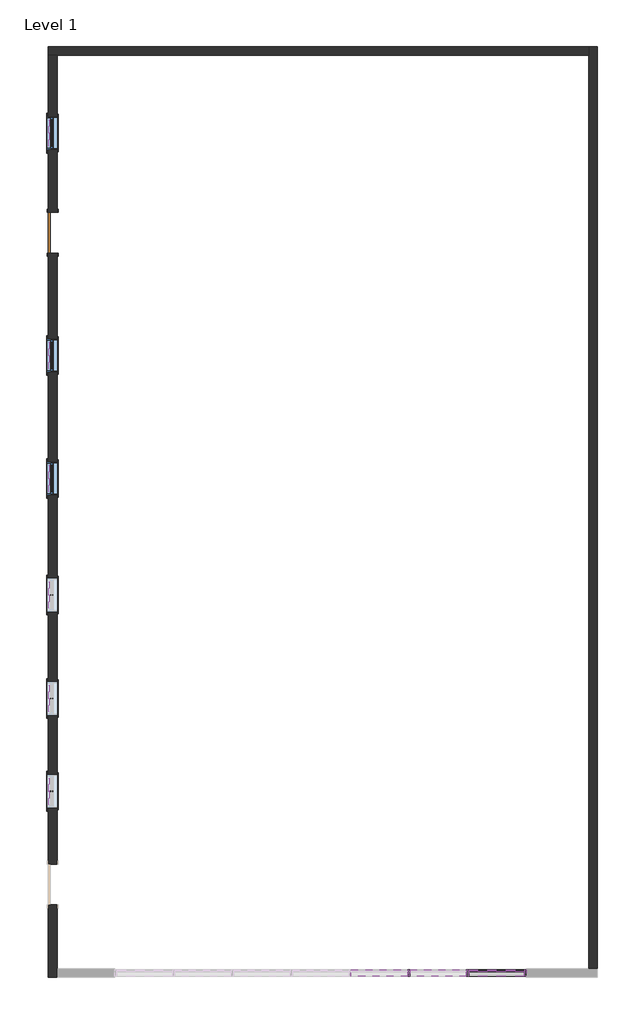
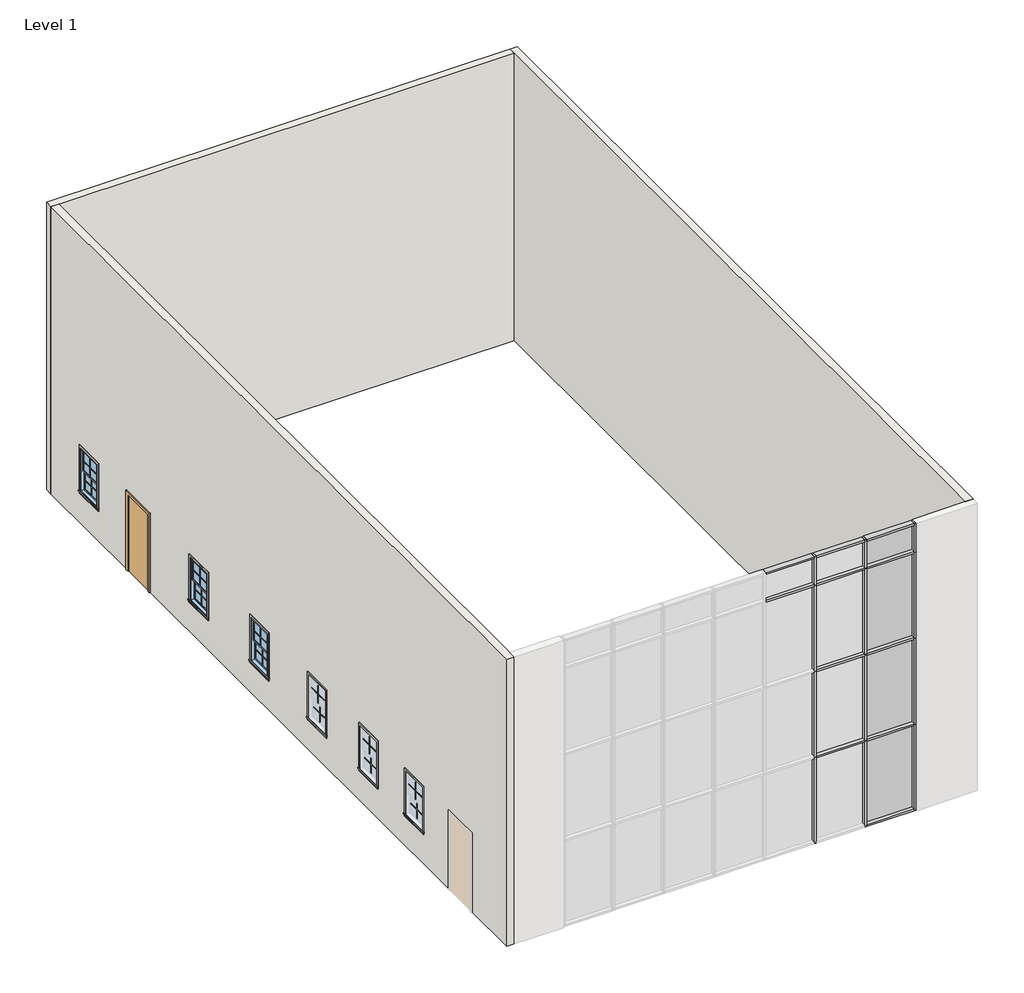
# One storey, part 2 of 2: 24 proxies, 23 members, 4 plates, 3 walls, 3 windows, 1 door.
"""IFC4 building model written with IfcOpenShell, lengths in millimetres."""

import ifcopenshell
import ifcopenshell.guid

model = None  # the IFC model being written
_history = None  # IfcOwnerHistory: only IFC2X3 demands one
_inside = {}  # id of a spatial element -> (the spatial element, [elements in it])
_under = {}  # id of a project, library or spatial element -> (it, [spatial elements below it])
_declared = {}  # id of a project -> (the project, [libraries it declares])
_typed = {}  # id of a type object -> (the type object, [elements of that type])
_made_of = {}  # id of a material, layer set ... -> (it, [elements and type objects made of it])


def new_model(schema):
    """Start an empty IFC model of exactly this schema.

    Asked for "IFC4X3", IfcOpenShell would pick the latest addendum, in which some entities
    have other attributes; the version numbers below select the first issue.
    IFC2X3 requires an IfcOwnerHistory on every rooted entity: one is made here for all.
    """
    global model, _history
    if schema == "IFC4X3":
        model = ifcopenshell.file(schema_version=(4, 3, 0, 0))
    else:
        model = ifcopenshell.file(schema=schema)
    _inside.clear()
    _under.clear()
    _declared.clear()
    _typed.clear()
    _made_of.clear()
    _history = None
    if model.schema == "IFC2X3":
        org = make("IfcOrganization", Name="unknown")
        user = make(
            "IfcPersonAndOrganization",
            ThePerson=make("IfcPerson", FamilyName="unknown"),
            TheOrganization=org,
        )
        app = make(
            "IfcApplication",
            ApplicationDeveloper=org,
            Version="unknown",
            ApplicationFullName="unknown",
            ApplicationIdentifier="unknown",
        )
        _history = make(
            "IfcOwnerHistory",
            OwningUser=user,
            OwningApplication=app,
            ChangeAction="ADDED",
            CreationDate=0,
        )
    return model


def make(cls, **values):
    """One entity of the class cls with the attributes given. An attribute that is None is left unset."""
    return model.create_entity(
        cls, **{name: value for name, value in values.items() if value is not None}
    )


def rooted(cls, **values):
    """An entity with a GlobalId (a new one), such as an element, a storey or a relation."""
    return make(cls, GlobalId=ifcopenshell.guid.new(), OwnerHistory=_history, **values)


def si_unit(unit_type, name, prefix=None):
    """IfcSIUnit, for example si_unit("LENGTHUNIT", "METRE", prefix="MILLI")."""
    return make("IfcSIUnit", UnitType=unit_type, Prefix=prefix, Name=name)


def assignment(units):
    """IfcUnitAssignment: the units of a project."""
    return None if units is None else make("IfcUnitAssignment", Units=units)


def point(xyz):
    """IfcCartesianPoint."""
    return None if xyz is None else make("IfcCartesianPoint", Coordinates=xyz)


def direction(xyz):
    """IfcDirection."""
    return None if xyz is None else make("IfcDirection", DirectionRatios=xyz)


def frame(location, z_axis=None, x_axis=None):
    """IfcAxis2Placement3D, a coordinate frame: its origin and axes. An axis left out is left unset."""
    return make(
        "IfcAxis2Placement3D",
        Location=point(location),
        Axis=direction(z_axis),
        RefDirection=direction(x_axis),
    )


def origin():
    """The frame at (0, 0, 0) with its axes left unset."""
    return frame((0.0, 0.0, 0.0))


def origin_with_axes():
    """The frame at (0, 0, 0) with the z axis (0, 0, 1) and the x axis (1, 0, 0) written out."""
    return frame((0.0, 0.0, 0.0), z_axis=(0.0, 0.0, 1.0), x_axis=(1.0, 0.0, 0.0))


def place(relative_to, where):
    """IfcLocalPlacement: puts the frame where relative to a parent placement (None: the world)."""
    return make(
        "IfcLocalPlacement", PlacementRelTo=relative_to, RelativePlacement=where
    )


def context(
    kind, dimensions, precision=None, world=None, true_north=None, identifier=None
):
    """IfcGeometricRepresentationContext, for example the 3D "Model" context."""
    return make(
        "IfcGeometricRepresentationContext",
        ContextIdentifier=identifier,
        ContextType=kind,
        CoordinateSpaceDimension=dimensions,
        Precision=precision,
        WorldCoordinateSystem=world,
        TrueNorth=true_north,
    )


def project(units=None, contexts=None):
    """IfcProject with its units and contexts."""
    return rooted(
        "IfcProject",
        Name="project",
        RepresentationContexts=contexts,
        UnitsInContext=assignment(units),
    )


def spatial(cls, under=None, at=None, **own):
    """A site, building, storey or space (cls), placed at a placement, below another one or the project."""
    s = rooted(cls, ObjectPlacement=at, **own)
    if under is not None:
        _under.setdefault(under.id(), (under, []))[1].append(s)
    return s


def polyline(points):
    """IfcPolyline through the points."""
    return make("IfcPolyline", Points=[point(p) for p in points])


def outline(outer, holes=None, kind="AREA"):
    """IfcArbitraryClosedProfileDef: a profile drawn as a closed curve; with holes, ...WithVoids."""
    if holes is None:
        return make("IfcArbitraryClosedProfileDef", ProfileType=kind, OuterCurve=outer)
    return make(
        "IfcArbitraryProfileDefWithVoids",
        ProfileType=kind,
        OuterCurve=outer,
        InnerCurves=holes,
    )


def extrude(swept, where, along, depth):
    """IfcExtrudedAreaSolid: the profile swept, set in the frame where, extruded along a direction by depth."""
    return make(
        "IfcExtrudedAreaSolid",
        SweptArea=swept,
        Position=where,
        ExtrudedDirection=direction(along),
        Depth=depth,
    )


def faces_of(points, faces, orient=None, outer=None):
    """IfcFace entities. A face is a list of loops; a loop is a list of indices into points, from 0.

    orient and outer hold one flag for each loop. By default every Orientation is true, the
    first loop of a face is its IfcFaceOuterBound and the others are IfcFaceBound.
    """
    made = []
    for i, loops in enumerate(faces):
        bounds = []
        for j, loop in enumerate(loops):
            is_outer = j == 0 if outer is None else outer[i][j]
            bounds.append(
                make(
                    "IfcFaceOuterBound" if is_outer else "IfcFaceBound",
                    Bound=make("IfcPolyLoop", Polygon=[points[k] for k in loop]),
                    Orientation=True if orient is None else orient[i][j],
                )
            )
        made.append(make("IfcFace", Bounds=bounds))
    return made


def faceted_brep(points, faces, orient=None, outer=None, voids=None):
    """IfcFacetedBrep: a solid bounded by flat faces; with voids (closed shells), ...WithVoids."""
    shared = [point(p) for p in points]
    hull = make("IfcClosedShell", CfsFaces=faces_of(shared, faces, orient, outer))
    if voids is None:
        return make("IfcFacetedBrep", Outer=hull)
    return make(
        "IfcFacetedBrepWithVoids",
        Outer=hull,
        Voids=[
            make(cls, CfsFaces=faces_of(shared, fs, o, b)) for cls, fs, o, b in voids
        ],
    )


def shape(context_of_items, identifier, shape_type, items):
    """IfcShapeRepresentation: the items that make up one representation, for example the "Body"."""
    return make(
        "IfcShapeRepresentation",
        ContextOfItems=context_of_items,
        RepresentationIdentifier=identifier,
        RepresentationType=shape_type,
        Items=items,
    )


def source(mapping_origin, context_of_items, identifier, shape_type, items):
    """IfcRepresentationMap: a shape defined once, which mapped items show again and again."""
    return make(
        "IfcRepresentationMap",
        MappingOrigin=mapping_origin,
        MappedRepresentation=shape(context_of_items, identifier, shape_type, items),
    )


def transform(
    local_origin,
    x_axis=None,
    y_axis=None,
    z_axis=None,
    scale=None,
    scale2=None,
    scale3=None,
    uniform=True,
):
    """IfcCartesianTransformationOperator3D, or its non-uniform kind. x_axis, y_axis, z_axis: its Axis1, 2, 3."""
    if uniform:
        return make(
            "IfcCartesianTransformationOperator3D",
            Axis1=direction(x_axis),
            Axis2=direction(y_axis),
            LocalOrigin=point(local_origin),
            Scale=scale,
            Axis3=direction(z_axis),
        )
    return make(
        "IfcCartesianTransformationOperator3DnonUniform",
        Axis1=direction(x_axis),
        Axis2=direction(y_axis),
        LocalOrigin=point(local_origin),
        Scale=scale,
        Axis3=direction(z_axis),
        Scale2=scale2,
        Scale3=scale3,
    )


def mapped(mapping_source, mapping_target):
    """IfcMappedItem: shows the shape of a source again, moved by a transform."""
    return make(
        "IfcMappedItem", MappingSource=mapping_source, MappingTarget=mapping_target
    )


def made_of(thing, what):
    """Note that an element or type object is made of a material, layer set ...; save() writes the relation."""
    if what is not None:
        _made_of.setdefault(what.id(), (what, []))[1].append(thing)
    return thing


def element(
    cls,
    number,
    at=None,
    inside=None,
    cuts=None,
    type_object=None,
    material=None,
    context=None,
    identifier="Body",
    shape_type=None,
    held_by="IfcProductDefinitionShape",
    body=None,
    shapes=None,
    **own,
):
    """One element of the class cls, such as IfcWall. Its Tag is "e" and its number.

    at: its placement. inside: the storey or other place that contains it. cuts: it is an
    opening in that element (IfcRelVoidsElement). A single representation is given by context,
    identifier, shape_type and body (its items); several are given by shapes. held_by: the class
    of the entity that holds the representations. save() writes the other relations.
    """
    e = rooted(cls, Tag="e%d" % number, ObjectPlacement=at, **own)
    if body is not None:
        shapes = [shape(context, identifier, shape_type, body)]
    if shapes is not None:
        e.Representation = make(held_by, Representations=shapes)
    if inside is not None:
        _inside.setdefault(inside.id(), (inside, []))[1].append(e)
    if cuts is not None:
        rooted(
            "IfcRelVoidsElement", RelatingBuildingElement=cuts, RelatedOpeningElement=e
        )
    if type_object is not None:
        _typed.setdefault(type_object.id(), (type_object, []))[1].append(e)
    return made_of(e, material)


def aggregate(whole, parts):
    """IfcRelAggregates: a whole, such as a stair, and the parts it consists of."""
    return rooted("IfcRelAggregates", RelatingObject=whole, RelatedObjects=parts)


def save(model, path):
    """Write the relations noted so far, then the file.

    IfcRelAggregates (storeys below a building ...), IfcRelContainedInSpatialStructure (elements
    in a storey), IfcRelDefinesByType, IfcRelAssociatesMaterial and IfcRelDeclares: one each for
    every whole, place, type object, material and project.
    """
    for whole, parts in _under.values():
        aggregate(whole, parts)
    for where, things in _inside.values():
        rooted(
            "IfcRelContainedInSpatialStructure",
            RelatedElements=things,
            RelatingStructure=where,
        )
    for kind, things in _typed.values():
        rooted("IfcRelDefinesByType", RelatedObjects=things, RelatingType=kind)
    for what, things in _made_of.values():
        rooted("IfcRelAssociatesMaterial", RelatedObjects=things, RelatingMaterial=what)
    for by, libraries in _declared.values():
        rooted("IfcRelDeclares", RelatingContext=by, RelatedDefinitions=libraries)
    model.write(path)


def m_muntin_pattern_2x2_m_muntin_pattern_2x2_aaec3afb(model_context):
    return source(origin(), model_context, "Body", "SweptSolid", [
        extrude(outline(polyline([(257.1375, -6.35), (257.1375, -298.8), (244.4375, -298.8), (244.4375, -6.35), (0.0, -6.35), (0.0, 6.35), (244.4375, 6.35), (244.4375, 298.8), (257.1375, 298.8), (257.1375, 6.35), (501.575, 6.35), (501.575, -6.35), (257.1375, -6.35)])), frame((0.0, 9.525, 0.0), z_axis=(0.0, 1.0, 0.0), x_axis=(0.0, 0.0, 1.0)), (0.0, 0.0, 1.0), 12.7),
        extrude(outline(polyline([(257.1375, -6.35), (257.1375, -298.8), (244.4375, -298.8), (244.4375, -6.35), (0.0, -6.35), (0.0, 6.35), (244.4375, 6.35), (244.4375, 298.8), (257.1375, 298.8), (257.1375, 6.35), (501.575, 6.35), (501.575, -6.35), (257.1375, -6.35)])), frame((0.0, -22.225, 0.0), z_axis=(0.0, 1.0, 0.0), x_axis=(0.0, 0.0, 1.0)), (0.0, 0.0, 1.0), 12.7),
    ])


def m_trim_window_exterior_flat_with_sill_e7ff6350(model_context):
    return source(origin(), model_context, "Body", "SweptSolid", [
        extrude(outline(polyline([(435.0, -1220.4323709), (435.0, -1280.4323709), (-435.0, -1280.4323709), (-435.0, -1220.4323709), (435.0, -1220.4323709)])), origin_with_axes(), (0.0, 0.0, 1.0), 19.05),
        extrude(outline(polyline([(-1230.0, 38.1), (-1202.4580645, 38.1), (-1200.0, 19.05), (-1200.0, 0.0), (-1220.4323709, 0.0), (-1220.4323709, 19.05), (-1230.0, 19.05), (-1230.0, 38.1)])), frame((-447.7, 0.0, 0.0), z_axis=(1.0, 0.0, 0.0), x_axis=(0.0, 1.0, 0.0)), (0.0, 0.0, 1.0), 895.4),
        extrude(outline(polyline([(-435.0, 60.0), (435.0, 60.0), (435.0, -1200.0), (375.0, -1200.0), (375.0, 0.0), (-375.0, 0.0), (-375.0, -1200.0), (-435.0, -1200.0), (-435.0, 60.0)])), origin_with_axes(), (0.0, 0.0, 1.0), 19.05),
    ])


def m_trim_window_interior_flat_picture_frame_31bd2320(model_context):
    return source(origin(), model_context, "Body", "SweptSolid", [
        extrude(outline(polyline([(422.3, 47.3), (422.3, -1247.3), (-422.3, -1247.3), (-422.3, 47.3), (422.3, 47.3)]), holes=[polyline([(362.3, -12.7), (-362.3, -12.7), (-362.3, -1187.3), (362.3, -1187.3), (362.3, -12.7)])]), origin_with_axes(), (0.0, 0.0, 1.0), 30.0),
    ])


def m_single_flush_0915_x_2134mm_6a9e8738(model_context):
    return source(origin(), model_context, "Body", "SweptSolid", [
        extrude(outline(polyline([(2210.0, -533.5), (0.0, -533.5), (0.0, -457.5), (2134.0, -457.5), (2134.0, 457.5), (0.0, 457.5), (0.0, 533.5), (2210.0, 533.5), (2210.0, -533.5)])), frame((0.0, 100.0, 0.0), z_axis=(0.0, 1.0, 0.0), x_axis=(0.0, 0.0, 1.0)), (0.0, 0.0, 1.0), 25.0),
        extrude(outline(polyline([(2210.0, 533.5), (2210.0, -533.5), (0.0, -533.5), (0.0, -457.5), (2134.0, -457.5), (2134.0, 457.5), (0.0, 457.5), (0.0, 533.5), (2210.0, 533.5)])), frame((0.0, -125.0, 0.0), z_axis=(0.0, 1.0, 0.0), x_axis=(0.0, 0.0, 1.0)), (0.0, 0.0, 1.0), 25.0),
        extrude(outline(polyline([(457.5, 49.0), (-457.5, 49.0), (-457.5, 100.0), (457.5, 100.0), (457.5, 49.0)])), origin_with_axes(), (0.0, 0.0, 1.0), 2134.0),
    ])


def rectangular_mullion_50mm_x_150mm_302a0cfa(model_context):
    return source(origin(), model_context, "Body", "SweptSolid", [
        extrude(outline(polyline([(0.0, 75.0), (0.0, -75.0), (-50.0, -75.0), (-50.0, 75.0), (0.0, 75.0)])), frame((0.0, 0.0, -1253.5714288), z_axis=(0.0, 0.0, 1.0), x_axis=(1.0, 0.0, 0.0)), (0.0, 0.0, 1.0), 1253.5714288),
    ])


def rectangular_mullion_50mm_x_150mm_46426fc7(model_context):
    return source(origin(), model_context, "Body", "SweptSolid", [
        extrude(outline(polyline([(25.0, 75.0), (25.0, -75.0), (-25.0, -75.0), (-25.0, 75.0), (25.0, 75.0)])), frame((0.0, 0.0, -1253.5714288), z_axis=(0.0, 0.0, 1.0), x_axis=(1.0, 0.0, 0.0)), (0.0, 0.0, 1.0), 1253.5714288),
    ])


def rectangular_mullion_50mm_x_150mm_f38f42f6(model_context):
    return source(origin(), model_context, "Body", "SweptSolid", [
        extrude(outline(polyline([(25.0, 75.0), (25.0, -75.0), (-25.0, -75.0), (-25.0, 75.0), (25.0, 75.0)])), frame((0.0, 0.0, -1278.5714285), z_axis=(0.0, 0.0, 1.0), x_axis=(1.0, 0.0, 0.0)), (0.0, 0.0, 1.0), 1278.5714285),
    ])


def rectangular_mullion_50mm_x_150mm_6225e4e3(model_context):
    return source(origin(), model_context, "Body", "SweptSolid", [
        extrude(outline(polyline([(25.0, 75.0), (25.0, -75.0), (-25.0, -75.0), (-25.0, 75.0), (25.0, 75.0)])), frame((0.0, 0.0, -2400.0), z_axis=(0.0, 0.0, 1.0), x_axis=(1.0, 0.0, 0.0)), (0.0, 0.0, 1.0), 2400.0),
    ])


def rectangular_mullion_50mm_x_150mm_662c37b1(model_context):
    return source(origin(), model_context, "Body", "SweptSolid", [
        extrude(outline(polyline([(0.0, 75.0), (0.0, -75.0), (-50.0, -75.0), (-50.0, 75.0), (0.0, 75.0)])), frame((0.0, 0.0, -2400.0), z_axis=(0.0, 0.0, 1.0), x_axis=(1.0, 0.0, 0.0)), (0.0, 0.0, 1.0), 2400.0),
    ])


def rectangular_mullion_50mm_x_150mm_14f10ac7(model_context):
    return source(origin(), model_context, "Body", "SweptSolid", [
        extrude(outline(polyline([(25.0, 75.0), (25.0, -75.0), (-25.0, -75.0), (-25.0, 75.0), (25.0, 75.0)])), frame((0.0, 0.0, -800.0), z_axis=(0.0, 0.0, 1.0), x_axis=(1.0, 0.0, 0.0)), (0.0, 0.0, 1.0), 800.0),
    ])


def rectangular_mullion_50mm_x_150mm_11a5ee59(model_context):
    return source(origin(), model_context, "Body", "SweptSolid", [
        extrude(outline(polyline([(0.0, 75.0), (0.0, -75.0), (-50.0, -75.0), (-50.0, 75.0), (0.0, 75.0)])), frame((0.0, 0.0, -1278.5714285), z_axis=(0.0, 0.0, 1.0), x_axis=(1.0, 0.0, 0.0)), (0.0, 0.0, 1.0), 1278.5714285),
    ])


def rectangular_mullion_50mm_x_150mm_6ffebc0f(model_context):
    return source(origin(), model_context, "Body", "SweptSolid", [
        extrude(outline(polyline([(0.0, 75.0), (0.0, -75.0), (-50.0, -75.0), (-50.0, 75.0), (0.0, 75.0)])), frame((0.0, 0.0, -800.0), z_axis=(0.0, 0.0, 1.0), x_axis=(1.0, 0.0, 0.0)), (0.0, 0.0, 1.0), 800.0),
    ])


def system_panel_glazed_b60b372a(model_context):
    return source(origin(), model_context, "Body", "SweptSolid", [
        extrude(outline(polyline([(626.7857144, 24.5), (-626.7857144, 24.5), (-626.7857144, 49.5), (626.7857144, 49.5), (626.7857144, 24.5)])), origin_with_axes(), (0.0, 0.0, 1.0), 2325.0),
    ])


def system_panel_glazed_eec4e8b3(model_context):
    return source(origin(), model_context, "Body", "SweptSolid", [
        extrude(outline(polyline([(626.7857144, 24.5), (-626.7857144, 24.5), (-626.7857144, 49.5), (626.7857144, 49.5), (626.7857144, 24.5)])), origin_with_axes(), (0.0, 0.0, 1.0), 2350.0),
    ])


def system_panel_glazed_efd17426(model_context):
    return source(origin(), model_context, "Body", "SweptSolid", [
        extrude(outline(polyline([(626.7857144, 24.5), (-626.7857144, 24.5), (-626.7857144, 49.5), (626.7857144, 49.5), (626.7857144, 24.5)])), origin_with_axes(), (0.0, 0.0, 1.0), 725.0),
    ])


def m_window_double_hung_750_x_1200mm_41070976(model_context):
    return source(origin(), model_context, "Body", "SweptSolid", [
        extrude(outline(polyline([(298.8, 30.15), (298.8, 23.8), (-298.8, 23.8), (-298.8, 30.15), (298.8, 30.15)])), frame((0.0, 0.0, 990.6), z_axis=(0.0, 0.0, 1.0), x_axis=(1.0, 0.0, 0.0)), (0.0, 0.0, 1.0), 501.575),
        extrude(outline(polyline([(-298.8, 17.45), (298.8, 17.45), (298.8, 11.1), (-298.8, 11.1), (-298.8, 17.45)])), frame((0.0, 0.0, 990.6), z_axis=(0.0, 0.0, 1.0), x_axis=(1.0, 0.0, 0.0)), (0.0, 0.0, 1.0), 501.575),
        extrude(outline(polyline([(298.8, 74.6), (298.8, 68.25), (-298.8, 68.25), (-298.8, 74.6), (298.8, 74.6)])), frame((0.0, 0.0, 1536.625), z_axis=(0.0, 0.0, 1.0), x_axis=(1.0, 0.0, 0.0)), (0.0, 0.0, 1.0), 501.575),
        extrude(outline(polyline([(-298.8, 61.9), (298.8, 61.9), (298.8, 55.55), (-298.8, 55.55), (-298.8, 61.9)])), frame((0.0, 0.0, 1536.625), z_axis=(0.0, 0.0, 1.0), x_axis=(1.0, 0.0, 0.0)), (0.0, 0.0, 1.0), 501.575),
        extrude(outline(polyline([(1536.625, -343.25), (946.15, -343.25), (946.15, 343.25), (1536.625, 343.25), (1536.625, -343.25)]), holes=[polyline([(1492.175, 298.8), (990.6, 298.8), (990.6, -298.8), (1492.175, -298.8), (1492.175, 298.8)])]), frame((0.0, -1.6, 0.0), z_axis=(0.0, 1.0, 0.0), x_axis=(0.0, 0.0, 1.0)), (0.0, 0.0, 1.0), 44.45),
        extrude(outline(polyline([(2082.65, -343.25), (1492.175, -343.25), (1492.175, 343.25), (2082.65, 343.25), (2082.65, -343.25)]), holes=[polyline([(2038.2, 298.8), (1536.625, 298.8), (1536.625, -298.8), (2038.2, -298.8), (2038.2, 298.8)])]), frame((0.0, 42.85, 0.0), z_axis=(0.0, 1.0, 0.0), x_axis=(0.0, 0.0, 1.0)), (0.0, 0.0, 1.0), 44.45),
        extrude(outline(polyline([(2114.4, -375.0), (914.4, -375.0), (914.4, 375.0), (2114.4, 375.0), (2114.4, -375.0)]), holes=[polyline([(2082.65, 343.25), (946.15, 343.25), (946.15, -343.25), (2082.65, -343.25), (2082.65, 343.25)])]), frame((0.0, -14.3, 0.0), z_axis=(0.0, 1.0, 0.0), x_axis=(0.0, 0.0, 1.0)), (0.0, 0.0, 1.0), 133.35),
        extrude(outline(polyline([(2114.4, 375.0), (2114.4, -375.0), (914.4, -375.0), (914.4, 375.0), (2114.4, 375.0)]), holes=[polyline([(2095.35, 355.95), (933.45, 355.95), (933.45, -355.95), (2095.35, -355.95), (2095.35, 355.95)])]), frame((0.0, -100.0, 0.0), z_axis=(0.0, 1.0, 0.0), x_axis=(0.0, 0.0, 1.0)), (0.0, 0.0, 1.0), 85.7),
    ])


model = new_model("IFC4")

# Units and contexts
model_context = context("Model", 3, world=origin())
ifc_project = project(units=[si_unit("LENGTHUNIT", "METRE", prefix="MILLI")], contexts=[model_context])

# Site, building, storey
site = spatial("IfcSite", under=ifc_project)
building = spatial("IfcBuilding", under=site)
storey = spatial("IfcBuildingStorey", under=building, Name="Level 1", Elevation=0.0)

# Proxies
placement = place(None, origin())
m_muntin_pattern_2x2_m_muntin_pattern_2x2_shape = m_muntin_pattern_2x2_m_muntin_pattern_2x2_aaec3afb(model_context)
element("IfcBuildingElementProxy", 1, Name="M_Muntin Pattern_2x2 : M_Muntin Pattern_2x2", ObjectType="M_Muntin Pattern_2x2 : M_Muntin Pattern_2x2", at=placement, inside=storey, context=model_context, shape_type="MappedRepresentation", body=[
    mapped(m_muntin_pattern_2x2_m_muntin_pattern_2x2_shape, transform((-7032.909392, -4566.9793434, 1536.625), x_axis=(0.0, 1.0, 0.0), y_axis=(-1.0, 0.0, 0.0), z_axis=(0.0, 0.0, 1.0))),
])
element("IfcBuildingElementProxy", 2, Name="M_Muntin Pattern_2x2 : M_Muntin Pattern_2x2", ObjectType="M_Muntin Pattern_2x2 : M_Muntin Pattern_2x2", at=placement, inside=storey, context=model_context, shape_type="MappedRepresentation", body=[
    mapped(m_muntin_pattern_2x2_m_muntin_pattern_2x2_shape, transform((-6988.459392, -4566.9793434, 990.6), x_axis=(0.0, 1.0, 0.0), y_axis=(-1.0, 0.0, 0.0), z_axis=(0.0, 0.0, 1.0))),
])
element("IfcBuildingElementProxy", 3, Name="M_Muntin Pattern_2x2 : M_Muntin Pattern_2x2", ObjectType="M_Muntin Pattern_2x2 : M_Muntin Pattern_2x2", at=placement, inside=storey, context=model_context, shape_type="MappedRepresentation", body=[
    mapped(m_muntin_pattern_2x2_m_muntin_pattern_2x2_shape, transform((-7032.909392, -2474.0000934, 1536.625), x_axis=(0.0, 1.0, 0.0), y_axis=(-1.0, 0.0, 0.0), z_axis=(0.0, 0.0, 1.0))),
])
element("IfcBuildingElementProxy", 4, Name="M_Muntin Pattern_2x2 : M_Muntin Pattern_2x2", ObjectType="M_Muntin Pattern_2x2 : M_Muntin Pattern_2x2", at=placement, inside=storey, context=model_context, shape_type="MappedRepresentation", body=[
    mapped(m_muntin_pattern_2x2_m_muntin_pattern_2x2_shape, transform((-6988.459392, -2474.0000934, 990.6), x_axis=(0.0, 1.0, 0.0), y_axis=(-1.0, 0.0, 0.0), z_axis=(0.0, 0.0, 1.0))),
])
element("IfcBuildingElementProxy", 5, Name="M_Muntin Pattern_2x2 : M_Muntin Pattern_2x2", ObjectType="M_Muntin Pattern_2x2 : M_Muntin Pattern_2x2", at=placement, inside=storey, context=model_context, shape_type="MappedRepresentation", body=[
    mapped(m_muntin_pattern_2x2_m_muntin_pattern_2x2_shape, transform((-7032.909392, -137.6511631, 1536.625), x_axis=(0.0, 1.0, 0.0), y_axis=(-1.0, 0.0, 0.0), z_axis=(0.0, 0.0, 1.0))),
])
element("IfcBuildingElementProxy", 6, Name="M_Muntin Pattern_2x2 : M_Muntin Pattern_2x2", ObjectType="M_Muntin Pattern_2x2 : M_Muntin Pattern_2x2", at=placement, inside=storey, context=model_context, shape_type="MappedRepresentation", body=[
    mapped(m_muntin_pattern_2x2_m_muntin_pattern_2x2_shape, transform((-6988.459392, -137.6511631, 990.6), x_axis=(0.0, 1.0, 0.0), y_axis=(-1.0, 0.0, 0.0), z_axis=(0.0, 0.0, 1.0))),
])
element("IfcBuildingElementProxy", 7, Name="M_Muntin Pattern_2x2 : M_Muntin Pattern_2x2", ObjectType="M_Muntin Pattern_2x2 : M_Muntin Pattern_2x2", at=placement, inside=storey, context=model_context, shape_type="MappedRepresentation", body=[
    mapped(m_muntin_pattern_2x2_m_muntin_pattern_2x2_shape, transform((-7032.909392, 2490.7413834, 1536.625), x_axis=(0.0, 1.0, 0.0), y_axis=(-1.0, 0.0, 0.0), z_axis=(0.0, 0.0, 1.0))),
])
element("IfcBuildingElementProxy", 8, Name="M_Muntin Pattern_2x2 : M_Muntin Pattern_2x2", ObjectType="M_Muntin Pattern_2x2 : M_Muntin Pattern_2x2", at=placement, inside=storey, context=model_context, shape_type="MappedRepresentation", body=[
    mapped(m_muntin_pattern_2x2_m_muntin_pattern_2x2_shape, transform((-6988.459392, 2490.7413834, 990.6), x_axis=(0.0, 1.0, 0.0), y_axis=(-1.0, 0.0, 0.0), z_axis=(0.0, 0.0, 1.0))),
])
element("IfcBuildingElementProxy", 9, Name="M_Muntin Pattern_2x2 : M_Muntin Pattern_2x2", ObjectType="M_Muntin Pattern_2x2 : M_Muntin Pattern_2x2", at=placement, inside=storey, context=model_context, shape_type="MappedRepresentation", body=[
    mapped(m_muntin_pattern_2x2_m_muntin_pattern_2x2_shape, transform((-7032.909392, 5265.1557382, 1536.625), x_axis=(0.0, 1.0, 0.0), y_axis=(-1.0, 0.0, 0.0), z_axis=(0.0, 0.0, 1.0))),
])
element("IfcBuildingElementProxy", 10, Name="M_Muntin Pattern_2x2 : M_Muntin Pattern_2x2", ObjectType="M_Muntin Pattern_2x2 : M_Muntin Pattern_2x2", at=placement, inside=storey, context=model_context, shape_type="MappedRepresentation", body=[
    mapped(m_muntin_pattern_2x2_m_muntin_pattern_2x2_shape, transform((-6988.459392, 5265.1557382, 990.6), x_axis=(0.0, 1.0, 0.0), y_axis=(-1.0, 0.0, 0.0), z_axis=(0.0, 0.0, 1.0))),
])
element("IfcBuildingElementProxy", 11, Name="M_Muntin Pattern_2x2 : M_Muntin Pattern_2x2", ObjectType="M_Muntin Pattern_2x2 : M_Muntin Pattern_2x2", at=placement, inside=storey, context=model_context, shape_type="MappedRepresentation", body=[
    mapped(m_muntin_pattern_2x2_m_muntin_pattern_2x2_shape, transform((-7032.909392, 10278.571151, 1536.625), x_axis=(0.0, 1.0, 0.0), y_axis=(-1.0, 0.0, 0.0), z_axis=(0.0, 0.0, 1.0))),
])
element("IfcBuildingElementProxy", 12, Name="M_Muntin Pattern_2x2 : M_Muntin Pattern_2x2", ObjectType="M_Muntin Pattern_2x2 : M_Muntin Pattern_2x2", at=placement, inside=storey, context=model_context, shape_type="MappedRepresentation", body=[
    mapped(m_muntin_pattern_2x2_m_muntin_pattern_2x2_shape, transform((-6988.459392, 10278.571151, 990.6), x_axis=(0.0, 1.0, 0.0), y_axis=(-1.0, 0.0, 0.0), z_axis=(0.0, 0.0, 1.0))),
])
m_trim_window_exterior_flat_with_sill_shape = m_trim_window_exterior_flat_with_sill_e7ff6350(model_context)
element("IfcBuildingElementProxy", 13, Name="M_Trim-Window-Exterior-Flat : with Sill", ObjectType="M_Trim-Window-Exterior-Flat : with Sill", at=placement, inside=storey, context=model_context, shape_type="MappedRepresentation", body=[
    mapped(m_trim_window_exterior_flat_with_sill_shape, transform((-7067.834392, -4566.9793434, 2114.4), x_axis=(0.0, -1.0, 0.0), y_axis=(0.0, 0.0, 1.0), z_axis=(-1.0, 0.0, 0.0))),
])
element("IfcBuildingElementProxy", 14, Name="M_Trim-Window-Exterior-Flat : with Sill", ObjectType="M_Trim-Window-Exterior-Flat : with Sill", at=placement, inside=storey, context=model_context, shape_type="MappedRepresentation", body=[
    mapped(m_trim_window_exterior_flat_with_sill_shape, transform((-7067.834392, -2474.0000934, 2114.4), x_axis=(0.0, -1.0, 0.0), y_axis=(0.0, 0.0, 1.0), z_axis=(-1.0, 0.0, 0.0))),
])
element("IfcBuildingElementProxy", 15, Name="M_Trim-Window-Exterior-Flat : with Sill", ObjectType="M_Trim-Window-Exterior-Flat : with Sill", at=placement, inside=storey, context=model_context, shape_type="MappedRepresentation", body=[
    mapped(m_trim_window_exterior_flat_with_sill_shape, transform((-7067.834392, -137.6511631, 2114.4), x_axis=(0.0, -1.0, 0.0), y_axis=(0.0, 0.0, 1.0), z_axis=(-1.0, 0.0, 0.0))),
])
element("IfcBuildingElementProxy", 16, Name="M_Trim-Window-Exterior-Flat : with Sill", ObjectType="M_Trim-Window-Exterior-Flat : with Sill", at=placement, inside=storey, context=model_context, shape_type="MappedRepresentation", body=[
    mapped(m_trim_window_exterior_flat_with_sill_shape, transform((-7067.834392, 2490.7413834, 2114.4), x_axis=(0.0, -1.0, 0.0), y_axis=(0.0, 0.0, 1.0), z_axis=(-1.0, 0.0, 0.0))),
])
element("IfcBuildingElementProxy", 17, Name="M_Trim-Window-Exterior-Flat : with Sill", ObjectType="M_Trim-Window-Exterior-Flat : with Sill", at=placement, inside=storey, context=model_context, shape_type="MappedRepresentation", body=[
    mapped(m_trim_window_exterior_flat_with_sill_shape, transform((-7067.834392, 5265.1557382, 2114.4), x_axis=(0.0, -1.0, 0.0), y_axis=(0.0, 0.0, 1.0), z_axis=(-1.0, 0.0, 0.0))),
])
element("IfcBuildingElementProxy", 18, Name="M_Trim-Window-Exterior-Flat : with Sill", ObjectType="M_Trim-Window-Exterior-Flat : with Sill", at=placement, inside=storey, context=model_context, shape_type="MappedRepresentation", body=[
    mapped(m_trim_window_exterior_flat_with_sill_shape, transform((-7067.834392, 10278.571151, 2114.4), x_axis=(0.0, -1.0, 0.0), y_axis=(0.0, 0.0, 1.0), z_axis=(-1.0, 0.0, 0.0))),
])
m_trim_window_interior_flat_picture_frame_shape = m_trim_window_interior_flat_picture_frame_31bd2320(model_context)
element("IfcBuildingElementProxy", 19, Name="M_Trim-Window-Interior-Flat : Picture Frame", ObjectType="M_Trim-Window-Interior-Flat : Picture Frame", at=placement, inside=storey, context=model_context, shape_type="MappedRepresentation", body=[
    mapped(m_trim_window_interior_flat_picture_frame_shape, transform((-6867.834392, -4566.9793434, 2114.4), x_axis=(0.0, 1.0, 0.0), y_axis=(0.0, 0.0, 1.0), z_axis=(1.0, 0.0, 0.0))),
])
element("IfcBuildingElementProxy", 20, Name="M_Trim-Window-Interior-Flat : Picture Frame", ObjectType="M_Trim-Window-Interior-Flat : Picture Frame", at=placement, inside=storey, context=model_context, shape_type="MappedRepresentation", body=[
    mapped(m_trim_window_interior_flat_picture_frame_shape, transform((-6867.834392, -2474.0000934, 2114.4), x_axis=(0.0, 1.0, 0.0), y_axis=(0.0, 0.0, 1.0), z_axis=(1.0, 0.0, 0.0))),
])
element("IfcBuildingElementProxy", 21, Name="M_Trim-Window-Interior-Flat : Picture Frame", ObjectType="M_Trim-Window-Interior-Flat : Picture Frame", at=placement, inside=storey, context=model_context, shape_type="MappedRepresentation", body=[
    mapped(m_trim_window_interior_flat_picture_frame_shape, transform((-6867.834392, -137.6511631, 2114.4), x_axis=(0.0, 1.0, 0.0), y_axis=(0.0, 0.0, 1.0), z_axis=(1.0, 0.0, 0.0))),
])
element("IfcBuildingElementProxy", 22, Name="M_Trim-Window-Interior-Flat : Picture Frame", ObjectType="M_Trim-Window-Interior-Flat : Picture Frame", at=placement, inside=storey, context=model_context, shape_type="MappedRepresentation", body=[
    mapped(m_trim_window_interior_flat_picture_frame_shape, transform((-6867.834392, 2490.7413834, 2114.4), x_axis=(0.0, 1.0, 0.0), y_axis=(0.0, 0.0, 1.0), z_axis=(1.0, 0.0, 0.0))),
])
element("IfcBuildingElementProxy", 23, Name="M_Trim-Window-Interior-Flat : Picture Frame", ObjectType="M_Trim-Window-Interior-Flat : Picture Frame", at=placement, inside=storey, context=model_context, shape_type="MappedRepresentation", body=[
    mapped(m_trim_window_interior_flat_picture_frame_shape, transform((-6867.834392, 5265.1557382, 2114.4), x_axis=(0.0, 1.0, 0.0), y_axis=(0.0, 0.0, 1.0), z_axis=(1.0, 0.0, 0.0))),
])
element("IfcBuildingElementProxy", 24, Name="M_Trim-Window-Interior-Flat : Picture Frame", ObjectType="M_Trim-Window-Interior-Flat : Picture Frame", at=placement, inside=storey, context=model_context, shape_type="MappedRepresentation", body=[
    mapped(m_trim_window_interior_flat_picture_frame_shape, transform((-6867.834392, 10278.571151, 2114.4), x_axis=(0.0, 1.0, 0.0), y_axis=(0.0, 0.0, 1.0), z_axis=(1.0, 0.0, 0.0))),
])

# Door
m_single_flush_0915_x_2134mm_shape = m_single_flush_0915_x_2134mm_6a9e8738(model_context)
element("IfcDoor", 25, ObjectType="M_Single-Flush : 0915 x 2134mm", at=placement, inside=storey, context=model_context, shape_type="MappedRepresentation", body=[
    mapped(m_single_flush_0915_x_2134mm_shape, transform((-6967.834392, 8033.0206566, 0.0), x_axis=(0.0, 1.0, 0.0), y_axis=(-1.0, 0.0, 0.0), z_axis=(0.0, 0.0, 1.0))),
])

# Members
rectangular_mullion_50mm_x_150mm_shape = rectangular_mullion_50mm_x_150mm_302a0cfa(model_context)
element("IfcMember", 26, ObjectType="Rectangular Mullion : 50mm x 150mm", at=placement, inside=storey, context=model_context, shape_type="MappedRepresentation", body=[
    mapped(rectangular_mullion_50mm_x_150mm_shape, transform((2428.5941792, -8666.9793434, 0.0), x_axis=(0.0, 0.0, -1.0), y_axis=(0.0, -1.0, 0.0), z_axis=(-1.0, 0.0, 0.0))),
])
rectangular_mullion_50mm_x_150mm_2_shape = rectangular_mullion_50mm_x_150mm_46426fc7(model_context)
element("IfcMember", 27, ObjectType="Rectangular Mullion : 50mm x 150mm", at=placement, inside=storey, context=model_context, shape_type="MappedRepresentation", body=[
    mapped(rectangular_mullion_50mm_x_150mm_2_shape, transform((3682.165608, -8666.9793434, 2400.0), x_axis=(0.0, 0.0, 1.0), y_axis=(0.0, -1.0, 0.0), z_axis=(1.0, 0.0, 0.0))),
])
element("IfcMember", 28, ObjectType="Rectangular Mullion : 50mm x 150mm", at=placement, inside=storey, context=model_context, shape_type="MappedRepresentation", body=[
    mapped(rectangular_mullion_50mm_x_150mm_2_shape, transform((3682.165608, -8666.9793434, 4800.0), x_axis=(0.0, 0.0, 1.0), y_axis=(0.0, -1.0, 0.0), z_axis=(1.0, 0.0, 0.0))),
])
element("IfcMember", 29, ObjectType="Rectangular Mullion : 50mm x 150mm", at=placement, inside=storey, context=model_context, shape_type="MappedRepresentation", body=[
    mapped(rectangular_mullion_50mm_x_150mm_2_shape, transform((3682.165608, -8666.9793434, 7200.0), x_axis=(0.0, 0.0, 1.0), y_axis=(0.0, -1.0, 0.0), z_axis=(1.0, 0.0, 0.0))),
])
rectangular_mullion_50mm_x_150mm_3_shape = rectangular_mullion_50mm_x_150mm_f38f42f6(model_context)
element("IfcMember", 30, ObjectType="Rectangular Mullion : 50mm x 150mm", at=placement, inside=storey, context=model_context, shape_type="MappedRepresentation", body=[
    mapped(rectangular_mullion_50mm_x_150mm_3_shape, transform((2378.5941792, -8666.9793434, 2400.0), x_axis=(0.0, 0.0, 1.0), y_axis=(0.0, -1.0, 0.0), z_axis=(1.0, 0.0, 0.0))),
])
element("IfcMember", 31, ObjectType="Rectangular Mullion : 50mm x 150mm", at=placement, inside=storey, context=model_context, shape_type="MappedRepresentation", body=[
    mapped(rectangular_mullion_50mm_x_150mm_3_shape, transform((2378.5941792, -8666.9793434, 4800.0), x_axis=(0.0, 0.0, 1.0), y_axis=(0.0, -1.0, 0.0), z_axis=(1.0, 0.0, 0.0))),
])
element("IfcMember", 32, ObjectType="Rectangular Mullion : 50mm x 150mm", at=placement, inside=storey, context=model_context, shape_type="MappedRepresentation", body=[
    mapped(rectangular_mullion_50mm_x_150mm_3_shape, transform((1050.0227508, -8666.9793434, 7200.0), x_axis=(0.0, 0.0, 1.0), y_axis=(0.0, -1.0, 0.0), z_axis=(1.0, 0.0, 0.0))),
])
element("IfcMember", 33, ObjectType="Rectangular Mullion : 50mm x 150mm", at=placement, inside=storey, context=model_context, shape_type="MappedRepresentation", body=[
    mapped(rectangular_mullion_50mm_x_150mm_3_shape, transform((2378.5941792, -8666.9793434, 7200.0), x_axis=(0.0, 0.0, 1.0), y_axis=(0.0, -1.0, 0.0), z_axis=(1.0, 0.0, 0.0))),
])
rectangular_mullion_50mm_x_150mm_4_shape = rectangular_mullion_50mm_x_150mm_6225e4e3(model_context)
element("IfcMember", 34, ObjectType="Rectangular Mullion : 50mm x 150mm", at=placement, inside=storey, context=model_context, shape_type="MappedRepresentation", body=[
    mapped(rectangular_mullion_50mm_x_150mm_4_shape, transform((1075.0227508, -8666.9793434, 0.0), x_axis=(1.0, 0.0, 0.0), y_axis=(0.0, -1.0, 0.0), z_axis=(0.0, 0.0, -1.0))),
])
element("IfcMember", 35, ObjectType="Rectangular Mullion : 50mm x 150mm", at=placement, inside=storey, context=model_context, shape_type="MappedRepresentation", body=[
    mapped(rectangular_mullion_50mm_x_150mm_4_shape, transform((2403.5941792, -8666.9793434, 0.0), x_axis=(1.0, 0.0, 0.0), y_axis=(0.0, -1.0, 0.0), z_axis=(0.0, 0.0, -1.0))),
])
element("IfcMember", 36, ObjectType="Rectangular Mullion : 50mm x 150mm", at=placement, inside=storey, context=model_context, shape_type="MappedRepresentation", body=[
    mapped(rectangular_mullion_50mm_x_150mm_4_shape, transform((1075.0227508, -8666.9793434, 2400.0), x_axis=(1.0, 0.0, 0.0), y_axis=(0.0, -1.0, 0.0), z_axis=(0.0, 0.0, -1.0))),
])
element("IfcMember", 37, ObjectType="Rectangular Mullion : 50mm x 150mm", at=placement, inside=storey, context=model_context, shape_type="MappedRepresentation", body=[
    mapped(rectangular_mullion_50mm_x_150mm_4_shape, transform((2403.5941792, -8666.9793434, 2400.0), x_axis=(1.0, 0.0, 0.0), y_axis=(0.0, -1.0, 0.0), z_axis=(0.0, 0.0, -1.0))),
])
element("IfcMember", 38, ObjectType="Rectangular Mullion : 50mm x 150mm", at=placement, inside=storey, context=model_context, shape_type="MappedRepresentation", body=[
    mapped(rectangular_mullion_50mm_x_150mm_4_shape, transform((1075.0227508, -8666.9793434, 4800.0), x_axis=(1.0, 0.0, 0.0), y_axis=(0.0, -1.0, 0.0), z_axis=(0.0, 0.0, -1.0))),
])
element("IfcMember", 39, ObjectType="Rectangular Mullion : 50mm x 150mm", at=placement, inside=storey, context=model_context, shape_type="MappedRepresentation", body=[
    mapped(rectangular_mullion_50mm_x_150mm_4_shape, transform((2403.5941792, -8666.9793434, 4800.0), x_axis=(1.0, 0.0, 0.0), y_axis=(0.0, -1.0, 0.0), z_axis=(0.0, 0.0, -1.0))),
])
rectangular_mullion_50mm_x_150mm_5_shape = rectangular_mullion_50mm_x_150mm_662c37b1(model_context)
element("IfcMember", 40, ObjectType="Rectangular Mullion : 50mm x 150mm", at=placement, inside=storey, context=model_context, shape_type="MappedRepresentation", body=[
    mapped(rectangular_mullion_50mm_x_150mm_5_shape, transform((3732.165608, -8666.9793434, 0.0), x_axis=(1.0, 0.0, 0.0), y_axis=(0.0, -1.0, 0.0), z_axis=(0.0, 0.0, -1.0))),
])
element("IfcMember", 41, ObjectType="Rectangular Mullion : 50mm x 150mm", at=placement, inside=storey, context=model_context, shape_type="MappedRepresentation", body=[
    mapped(rectangular_mullion_50mm_x_150mm_5_shape, transform((3732.165608, -8666.9793434, 2400.0), x_axis=(1.0, 0.0, 0.0), y_axis=(0.0, -1.0, 0.0), z_axis=(0.0, 0.0, -1.0))),
])
element("IfcMember", 42, ObjectType="Rectangular Mullion : 50mm x 150mm", at=placement, inside=storey, context=model_context, shape_type="MappedRepresentation", body=[
    mapped(rectangular_mullion_50mm_x_150mm_5_shape, transform((3732.165608, -8666.9793434, 4800.0), x_axis=(1.0, 0.0, 0.0), y_axis=(0.0, -1.0, 0.0), z_axis=(0.0, 0.0, -1.0))),
])
rectangular_mullion_50mm_x_150mm_6_shape = rectangular_mullion_50mm_x_150mm_14f10ac7(model_context)
element("IfcMember", 43, ObjectType="Rectangular Mullion : 50mm x 150mm", at=placement, inside=storey, context=model_context, shape_type="MappedRepresentation", body=[
    mapped(rectangular_mullion_50mm_x_150mm_6_shape, transform((1075.0227508, -8666.9793434, 7200.0), x_axis=(1.0, 0.0, 0.0), y_axis=(0.0, -1.0, 0.0), z_axis=(0.0, 0.0, -1.0))),
])
element("IfcMember", 44, ObjectType="Rectangular Mullion : 50mm x 150mm", at=placement, inside=storey, context=model_context, shape_type="MappedRepresentation", body=[
    mapped(rectangular_mullion_50mm_x_150mm_6_shape, transform((2403.5941792, -8666.9793434, 7200.0), x_axis=(1.0, 0.0, 0.0), y_axis=(0.0, -1.0, 0.0), z_axis=(0.0, 0.0, -1.0))),
])
element("IfcMember", 45, ObjectType="Rectangular Mullion : 50mm x 150mm", at=placement, inside=storey, context=model_context, shape_type="MappedRepresentation", body=[
    mapped(rectangular_mullion_50mm_x_150mm_shape, transform((3682.165608, -8666.9793434, 8000.0), x_axis=(0.0, 0.0, 1.0), y_axis=(0.0, -1.0, 0.0), z_axis=(1.0, 0.0, 0.0))),
])
rectangular_mullion_50mm_x_150mm_7_shape = rectangular_mullion_50mm_x_150mm_11a5ee59(model_context)
element("IfcMember", 46, ObjectType="Rectangular Mullion : 50mm x 150mm", at=placement, inside=storey, context=model_context, shape_type="MappedRepresentation", body=[
    mapped(rectangular_mullion_50mm_x_150mm_7_shape, transform((1050.0227508, -8666.9793434, 8000.0), x_axis=(0.0, 0.0, 1.0), y_axis=(0.0, -1.0, 0.0), z_axis=(1.0, 0.0, 0.0))),
])
element("IfcMember", 47, ObjectType="Rectangular Mullion : 50mm x 150mm", at=placement, inside=storey, context=model_context, shape_type="MappedRepresentation", body=[
    mapped(rectangular_mullion_50mm_x_150mm_7_shape, transform((2378.5941792, -8666.9793434, 8000.0), x_axis=(0.0, 0.0, 1.0), y_axis=(0.0, -1.0, 0.0), z_axis=(1.0, 0.0, 0.0))),
])
rectangular_mullion_50mm_x_150mm_8_shape = rectangular_mullion_50mm_x_150mm_6ffebc0f(model_context)
element("IfcMember", 48, ObjectType="Rectangular Mullion : 50mm x 150mm", at=placement, inside=storey, context=model_context, shape_type="MappedRepresentation", body=[
    mapped(rectangular_mullion_50mm_x_150mm_8_shape, transform((3732.165608, -8666.9793434, 7200.0), x_axis=(1.0, 0.0, 0.0), y_axis=(0.0, -1.0, 0.0), z_axis=(0.0, 0.0, -1.0))),
])

# Plates
system_panel_glazed_shape = system_panel_glazed_b60b372a(model_context)
element("IfcPlate", 49, ObjectType="System Panel : Glazed", at=placement, inside=storey, context=model_context, shape_type="MappedRepresentation", body=[
    mapped(system_panel_glazed_shape, transform((3055.3798936, -8666.9793434, 50.0), x_axis=(1.0, 0.0, 0.0), y_axis=(0.0, 1.0, 0.0), z_axis=(0.0, 0.0, 1.0))),
])
system_panel_glazed_2_shape = system_panel_glazed_eec4e8b3(model_context)
element("IfcPlate", 50, ObjectType="System Panel : Glazed", at=placement, inside=storey, context=model_context, shape_type="MappedRepresentation", body=[
    mapped(system_panel_glazed_2_shape, transform((3055.3798936, -8666.9793434, 2425.0), x_axis=(1.0, 0.0, 0.0), y_axis=(0.0, 1.0, 0.0), z_axis=(0.0, 0.0, 1.0))),
])
element("IfcPlate", 51, ObjectType="System Panel : Glazed", at=placement, inside=storey, context=model_context, shape_type="MappedRepresentation", body=[
    mapped(system_panel_glazed_2_shape, transform((3055.3798936, -8666.9793434, 4825.0), x_axis=(1.0, 0.0, 0.0), y_axis=(0.0, 1.0, 0.0), z_axis=(0.0, 0.0, 1.0))),
])
system_panel_glazed_3_shape = system_panel_glazed_efd17426(model_context)
element("IfcPlate", 52, ObjectType="System Panel : Glazed", at=placement, inside=storey, context=model_context, shape_type="MappedRepresentation", body=[
    mapped(system_panel_glazed_3_shape, transform((3055.3798936, -8666.9793434, 7225.0), x_axis=(1.0, 0.0, 0.0), y_axis=(0.0, 1.0, 0.0), z_axis=(0.0, 0.0, 1.0))),
])

# Walls
element("IfcWall", 53, ObjectType="Generic - 200mm", at=placement, inside=storey, context=model_context, shape_type="Brep", body=[
    faceted_brep([(-7067.834392, 12033.0206566, 0.0), (-6867.834392, 12033.0206566, 0.0), (5132.165608, 12033.0206566, 0.0), (5132.165608, 12033.0206566, 8000.0), (-6867.834392, 12033.0206566, 8000.0), (-7067.834392, 12033.0206566, 8000.0), (-7067.834392, 12233.0206566, 0.0), (-7067.834392, 12233.0206566, 8000.0), (5132.165608, 12233.0206566, 8000.0), (5132.165608, 12233.0206566, 0.0)], [[[0, 1, 2, 3, 4, 5]], [[6, 7, 8, 9]], [[2, 1, 0, 6, 9]], [[5, 4, 3, 8, 7]], [[0, 5, 7, 6]], [[3, 2, 9, 8]]]),
])
element("IfcWall", 54, ObjectType="Generic - 200mm", at=placement, inside=storey, context=model_context, shape_type="Brep", body=[
    faceted_brep([(-6867.834392, 12033.0206566, 8000.0), (-6867.834392, -8566.9793434, 8000.0), (-6867.834392, -8766.9793434, 8000.0), (-6867.834392, -8766.9793434, 0.0), (-6867.834392, -8566.9793434, 0.0), (-6867.834392, -7124.4793434, 0.0), (-6867.834392, -7124.4793434, 2134.0), (-6867.834392, -6209.4793434, 2134.0), (-6867.834392, -6209.4793434, 0.0), (-6867.834392, 7575.5206566, 0.0), (-6867.834392, 7575.5206566, 2134.0), (-6867.834392, 8490.5206566, 2134.0), (-6867.834392, 8490.5206566, 0.0), (-6867.834392, 12033.0206566, 0.0), (-6867.834392, -4941.9793434, 2114.4), (-6867.834392, -4191.9793434, 2114.4), (-6867.834392, -4191.9793434, 914.4), (-6867.834392, -4941.9793434, 914.4), (-6867.834392, -2849.0000934, 914.4), (-6867.834392, -2849.0000934, 2114.4), (-6867.834392, -2099.0000934, 2114.4), (-6867.834392, -2099.0000934, 914.4), (-6867.834392, -512.6511631, 914.4), (-6867.834392, -512.6511631, 2114.4), (-6867.834392, 237.3488369, 2114.4), (-6867.834392, 237.3488369, 914.4), (-6867.834392, 2115.7413834, 914.4), (-6867.834392, 2115.7413834, 2114.4), (-6867.834392, 2865.7413834, 2114.4), (-6867.834392, 2865.7413834, 914.4), (-6867.834392, 4890.1557382, 914.4), (-6867.834392, 4890.1557382, 2114.4), (-6867.834392, 5640.1557382, 2114.4), (-6867.834392, 5640.1557382, 914.4), (-6867.834392, 9903.571151, 914.4), (-6867.834392, 9903.571151, 2114.4), (-6867.834392, 10653.571151, 2114.4), (-6867.834392, 10653.571151, 914.4), (-7067.834392, -8766.9793434, 8000.0), (-7067.834392, 12033.0206566, 8000.0), (-7067.834392, 12033.0206566, 0.0), (-7067.834392, 8490.5206566, 0.0), (-7067.834392, 8490.5206566, 2134.0), (-7067.834392, 7575.5206566, 2134.0), (-7067.834392, 7575.5206566, 0.0), (-7067.834392, -6209.4793434, 0.0), (-7067.834392, -6209.4793434, 2134.0), (-7067.834392, -7124.4793434, 2134.0), (-7067.834392, -7124.4793434, 0.0), (-7067.834392, -8766.9793434, 0.0), (-7067.834392, -4941.9793434, 2114.4), (-7067.834392, -4941.9793434, 914.4), (-7067.834392, -4191.9793434, 914.4), (-7067.834392, -4191.9793434, 2114.4), (-7067.834392, -2849.0000934, 2114.4), (-7067.834392, -2849.0000934, 914.4), (-7067.834392, -2099.0000934, 914.4), (-7067.834392, -2099.0000934, 2114.4), (-7067.834392, -512.6511631, 2114.4), (-7067.834392, -512.6511631, 914.4), (-7067.834392, 237.3488369, 914.4), (-7067.834392, 237.3488369, 2114.4), (-7067.834392, 2115.7413834, 2114.4), (-7067.834392, 2115.7413834, 914.4), (-7067.834392, 2865.7413834, 914.4), (-7067.834392, 2865.7413834, 2114.4), (-7067.834392, 4890.1557382, 2114.4), (-7067.834392, 4890.1557382, 914.4), (-7067.834392, 5640.1557382, 914.4), (-7067.834392, 5640.1557382, 2114.4), (-7067.834392, 9903.571151, 2114.4), (-7067.834392, 9903.571151, 914.4), (-7067.834392, 10653.571151, 914.4), (-7067.834392, 10653.571151, 2114.4)], [[[0, 1, 2, 3, 4, 5, 6, 7, 8, 9, 10, 11, 12, 13], [14, 15, 16, 17], [18, 19, 20, 21], [22, 23, 24, 25], [26, 27, 28, 29], [30, 31, 32, 33], [34, 35, 36, 37]], [[38, 39, 40, 41, 42, 43, 44, 45, 46, 47, 48, 49], [50, 51, 52, 53], [54, 55, 56, 57], [58, 59, 60, 61], [62, 63, 64, 65], [66, 67, 68, 69], [70, 71, 72, 73]], [[3, 49, 48, 5, 4]], [[40, 13, 12, 41]], [[8, 45, 44, 9]], [[2, 1, 0, 39, 38]], [[3, 2, 38, 49]], [[0, 13, 40, 39]], [[46, 45, 8, 7]], [[47, 46, 7, 6]], [[48, 47, 6, 5]], [[42, 41, 12, 11]], [[43, 42, 11, 10]], [[44, 43, 10, 9]], [[51, 50, 14, 17]], [[52, 51, 17, 16]], [[53, 52, 16, 15]], [[50, 53, 15, 14]], [[54, 19, 18, 55]], [[55, 18, 21, 56]], [[56, 21, 20, 57]], [[19, 54, 57, 20]], [[58, 23, 22, 59]], [[59, 22, 25, 60]], [[60, 25, 24, 61]], [[23, 58, 61, 24]], [[62, 27, 26, 63]], [[63, 26, 29, 64]], [[64, 29, 28, 65]], [[27, 62, 65, 28]], [[66, 31, 30, 67]], [[67, 30, 33, 68]], [[68, 33, 32, 69]], [[31, 66, 69, 32]], [[70, 35, 34, 71]], [[71, 34, 37, 72]], [[72, 37, 36, 73]], [[35, 70, 73, 36]]]),
])
element("IfcWall", 55, ObjectType="Generic - 200mm", at=placement, inside=storey, context=model_context, shape_type="Brep", body=[
    faceted_brep([(5132.165608, 12233.0206566, 0.0), (5132.165608, 12033.0206566, 0.0), (5132.165608, -8566.9793434, 0.0), (5132.165608, -8566.9793434, 8000.0), (5132.165608, 12033.0206566, 8000.0), (5132.165608, 12233.0206566, 8000.0), (5332.165608, 12233.0206566, 0.0), (5332.165608, 12233.0206566, 8000.0), (5332.165608, -8566.9793434, 8000.0), (5332.165608, -8566.9793434, 0.0)], [[[0, 1, 2, 3, 4, 5]], [[6, 7, 8, 9]], [[2, 1, 0, 6, 9]], [[5, 4, 3, 8, 7]], [[0, 5, 7, 6]], [[3, 2, 9, 8]]]),
])

# Windows
m_window_double_hung_750_x_1200mm_shape = m_window_double_hung_750_x_1200mm_41070976(model_context)
element("IfcWindow", 56, ObjectType="M_Window-Double-Hung : 750 x 1200mm", at=placement, inside=storey, context=model_context, shape_type="MappedRepresentation", body=[
    mapped(m_window_double_hung_750_x_1200mm_shape, transform((-6967.834392, 2490.7413834, 0.0), x_axis=(0.0, 1.0, 0.0), y_axis=(-1.0, 0.0, 0.0), z_axis=(0.0, 0.0, 1.0))),
])
element("IfcWindow", 57, ObjectType="M_Window-Double-Hung : 750 x 1200mm", at=placement, inside=storey, context=model_context, shape_type="MappedRepresentation", body=[
    mapped(m_window_double_hung_750_x_1200mm_shape, transform((-6967.834392, 5265.1557382, 0.0), x_axis=(0.0, 1.0, 0.0), y_axis=(-1.0, 0.0, 0.0), z_axis=(0.0, 0.0, 1.0))),
])
element("IfcWindow", 58, ObjectType="M_Window-Double-Hung : 750 x 1200mm", at=placement, inside=storey, context=model_context, shape_type="MappedRepresentation", body=[
    mapped(m_window_double_hung_750_x_1200mm_shape, transform((-6967.834392, 10278.571151, 0.0), x_axis=(0.0, 1.0, 0.0), y_axis=(-1.0, 0.0, 0.0), z_axis=(0.0, 0.0, 1.0))),
])

save(model, "model.ifc")

# Revit data of these elements
# Type "M_Muntin Pattern_2x2 : M_Muntin Pattern_2x2"
#   Width [instance default] = 1200 mm
#   Thickness = 12.7 mm
#   Height [instance default] = 1200 mm
#   Distance = 19.05 mm
#   Interior Material [instance default] = none
#   Exterior Material [instance default] = none
#   Default Elevation = 0
# Type "M_Trim-Window-Exterior-Flat : with Sill"
#   Trim Width = 60 mm
#   Trim Thickness_Picture Frame = 30 mm
#   Trim Thickness_with Sill = 19.05 mm
#   Sill Thickness = 30 mm
#   Opening Width [instance default] = 600 mm
#   Opening Height [instance default] = 900 mm
#   Default Elevation = 1200 mm
#   Sill = yes
#   Picture Frame = no
#   Trim Material [instance default] = none
# Type "M_Trim-Window-Interior-Flat : Picture Frame"
#   Trim Thickness_Picture Frame = 30 mm
#   Trim Width = 60 mm
#   Trim Thickness_with Sill = 20 mm
#   Sill Thickness = 30 mm
#   Opening Width [instance default] = 600 mm
#   Opening Height [instance default] = 900 mm
#   Default Elevation = 1200 mm
#   Sill = no
#   Picture Frame = yes
#   Trim Material [instance default] = none
# Type "M_Single-Flush : 0915 x 2134mm"
#   Type Mark = "15"
#   Construction Type Id = "MDOOR"
#   Analytic Construction = "Metal"
#   Thickness = 51 mm
#   Thermal Resistance (R) = 0.270117 (m²·K)/W
#   Heat Transfer Coefficient (U) = 3.7021 W/(m²·K)
#   Height = 2134 mm
#   Trim Projection Ext = 25 mm
#   Trim Projection Int = 25 mm
#   Trim Width = 76 mm
#   Width = 915 mm
#   Define Thermal Properties by = 1
#   Door Material = Door - Panel
#   Frame Material = Door - Frame
#   Visual Light Transmittance = 0
#   Solar Heat Gain Coefficient = 0
#   Function = (empty or 0)
#   Wall Closure = (empty or 0)
# Type "Rectangular Mullion : 50mm x 150mm"
#   built-in parameter 1007304 = 0.492126 (stored number, unit not read)
#   built-in parameter 1007301 = 0.082021 (stored number, unit not read)
#   built-in parameter 1007300 = 0.082021 (stored number, unit not read)
# Type "System Panel : Glazed"
#   Construction Type Id = "GSP4R"
#   Analytic Construction = "1/8 in Pilkington single glazing"
#   Visual Light Transmittance = 0.9
#   Solar Heat Gain Coefficient = 0.86
#   Heat Transfer Coefficient (U) = 6.7069 W/(m²·K)
#   Define Thermal Properties by = 1
# Type "Generic - 200mm"
#   Layers, outside or top first: 200 mm no material (function 1)
# Type "M_Window-Double-Hung : 750 x 1200mm"
#   Type Mark = "26"
#   Fire Rating = "0.5h"
#   Construction Type Id = "DG-DR"
#   Assembly Code = "B2020100"
#   Analytic Construction = "Double glazing - domestic"
#   Wall Thickness [instance default] = 150 mm
#   Window Inset [instance default] = 0 mm
#   Visual Light Transmittance = 0.81
#   Thermal Resistance (R) = 0.319569 (m²·K)/W
#   Solar Heat Gain Coefficient = 0.76
#   Muntin Width = 597.6 mm
#   Muntin Height = 501.575 mm
#   Interior Wall Closure [instance default] = 35.7 mm
#   Rough Width = 765 mm
#   Rough Height = 1215 mm
#   Frame Extension [instance default] = 31.75 mm
#   Exterior Wall Closure [instance default] = 12.7 mm
#   Extension Jamb [instance default] = 35.7 mm
#   Heat Transfer Coefficient (U) = 3.12929 W/(m²·K)
#   Height = 1200 mm
#   Width = 750 mm
#   Define Thermal Properties by = 1
#   Top Muntin Visibility = yes
#   Indicator Visibility [instance default] = yes
#   Extension Jamb Visibility [instance default] = yes
#   Interior Trim Visibility [instance default] = yes
#   Exterior Trim Visibility [instance default] = yes
#   Bottom Muntin Visibility = yes
#   Muntin Pattern = M_Muntin Pattern_2x2 : M_Muntin Pattern_2x2
#   Interior Trim Material = Wood - Stained
#   Interior Trim = M_Trim-Window-Interior-Flat : Picture Frame
#   Exterior Trim Material = Clad - White
#   Exterior Trim = M_Trim-Window-Exterior-Flat : with Sill
#   Glass Panel Material = Glass
#   Exterior Frame Material = Clad - White
#   Interior Frame Material = Wood - Stained
#   Wall Closure = (empty or 0)
# Elements 1, 2, 3, 4, 5, 6, 7, 8, 9, 10, 11, 12 (IfcBuildingElementProxy, "M_Muntin Pattern_2x2 : M_Muntin Pattern_2x2")
#   Width = 597.6 mm
#   Height = 501.575 mm
#   Interior Material = Wood - Stained
#   Exterior Material = Clad - White
#   Phase Created = New Construction
#   Materials on its faces: "Clad - White", "Wood - Stained"
# Elements 13, 14, 15, 16, 17, 18 (IfcBuildingElementProxy, "M_Trim-Window-Exterior-Flat : with Sill")
#   Opening Width = 750 mm
#   Opening Height = 1200 mm
#   Trim Material = Clad - White
#   Phase Created = New Construction
#   Materials on its faces: "Clad - White"
# Elements 19, 20, 21, 22, 23, 24 (IfcBuildingElementProxy, "M_Trim-Window-Interior-Flat : Picture Frame")
#   Opening Width = 750 mm
#   Opening Height = 1200 mm
#   Trim Material = Wood - Stained
#   Phase Created = New Construction
#   Materials on its faces: "Wood - Stained"
# Element 25 (IfcDoor, "M_Single-Flush : 0915 x 2134mm")
#   Phase Created = New Construction
#   Materials on its faces: "Door - Frame", "Door - Panel"
# Elements 26, 27, 28, 29, 30, 31, 32, 33, 34, 35, 36, 37, 38, 39, 40, 41, 42, 43, 44, 45, 46, 47, 48 (IfcMember, "Rectangular Mullion : 50mm x 150mm")
#   Phase Created = New Construction
#   Materials on its faces: "Aluminum"
# Elements 49, 50, 51, 52 (IfcPlate, "System Panel : Glazed")
#   Phase Created = New Construction
#   Materials on its faces: "Glass"
# Elements 53, 54, 55 (IfcWall, "Generic - 200mm")
#   Top Offset = 0 mm
#   Base Offset = 0 mm
#   Unconnected Height = 8000 mm
#   wall height = 8000 mm
#   Phase Created = New Construction
#   Base Constraint = Level 1
#   Materials on its faces: "Default Wall"
# Element 56 (IfcWindow, "M_Window-Double-Hung : 750 x 1200mm")
#   Mark = "9"
#   Window Inset = 0 mm
#   Interior Wall Closure = 35.7 mm
#   Frame Extension = 31.75 mm
#   Exterior Wall Closure = 12.7 mm
#   Interior Trim Visibility = yes
#   Indicator Visibility = yes
#   Exterior Trim Visibility = yes
#   Phase Created = New Construction
#   Materials on its faces: "Wood - Stained", "Glass", "Clad - White"
# Element 57 (IfcWindow, "M_Window-Double-Hung : 750 x 1200mm")
#   Mark = "10"
#   Window Inset = 0 mm
#   Interior Wall Closure = 35.7 mm
#   Frame Extension = 31.75 mm
#   Exterior Wall Closure = 12.7 mm
#   Interior Trim Visibility = yes
#   Indicator Visibility = yes
#   Exterior Trim Visibility = yes
#   Phase Created = New Construction
#   Materials on its faces: "Wood - Stained", "Glass", "Clad - White"
# Element 58 (IfcWindow, "M_Window-Double-Hung : 750 x 1200mm")
#   Mark = "11"
#   Window Inset = 0 mm
#   Interior Wall Closure = 35.7 mm
#   Frame Extension = 31.75 mm
#   Exterior Wall Closure = 12.7 mm
#   Interior Trim Visibility = yes
#   Indicator Visibility = yes
#   Exterior Trim Visibility = yes
#   Phase Created = New Construction
#   Materials on its faces: "Wood - Stained", "Glass", "Clad - White"
# Materials
#   "Door - Panel": class "Wood", colour RGB 210 159 95, transparency 0, Cost = 0
#   "Door - Frame": class "Miscellaneous", colour RGB 118 70 51, transparency 0, Cost = 0
#   "Wood - Stained": class "Wood", colour RGB 227 170 128, transparency 0, Cost = 0
#   "Clad - White": class "Wood", colour RGB 242 242 238, transparency 0, Cost = 0
#   "Glass": class "Glass", colour RGB 0 128 192, transparency 0.75, Description = "Soda Lime Glass", Cost = 0
#   "Aluminum": class "Metal", colour RGB 247 247 247, transparency 0, Description = "Aluminum 6061", Cost = 0
#   "Default Wall": class "Miscellaneous", colour RGB 128 128 128, transparency 0, Cost = 0
